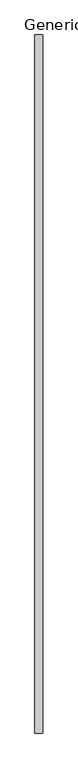
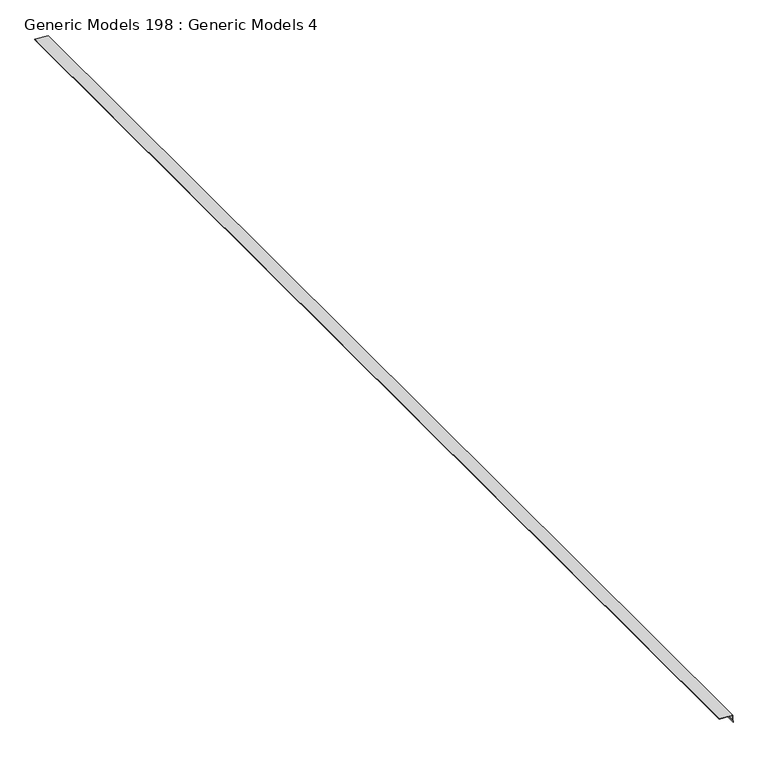
"""IFC4 building model written with IfcOpenShell, lengths in millimetres: proxy geometry, Generic Models 198 : Generic Models 4."""

from ifc_helpers import new_model, si_unit, frame, origin, place, context, project, spatial, polyline, outline, extrude, source, transform, mapped, element, save


def generic_models_198_generic_models_4_338ca49c(model_context):
    return source(origin(), model_context, "Body", "SweptSolid", [
        extrude(outline(polyline([(126852.2693751, -8160.3860198), (126833.2354151, -8160.3860198), (126833.2354151, -8159.5922698), (126852.4093346, -8159.5922698), (126859.5412752, -8162.1880839), (126925.6844476, -8162.1880839), (126932.2834421, -8320.5639511), (126931.4903802, -8320.5969953), (126924.9230818, -8162.9818339), (126859.4013156, -8162.9818339), (126852.2693751, -8160.3860198)])), frame((0.0, -6864.9230338, 0.0), z_axis=(0.0, 1.0, 0.0), x_axis=(0.0, 0.0, 1.0)), (0.0, 0.0, 1.0), 13919.2),
    ])


if __name__ == "__main__":
    model = new_model("IFC4")
    model_context = context("Model", 3, world=origin())
    ifc_project = project(units=[si_unit("LENGTHUNIT", "METRE", prefix="MILLI")], contexts=[model_context])
    site = spatial("IfcSite", under=ifc_project)
    building = spatial("IfcBuilding", under=site)
    placement = place(None, origin())
    generic_models_198_generic_models_4_shape = generic_models_198_generic_models_4_338ca49c(model_context)
    element("IfcBuildingElementProxy", 1, Name="Generic Models 198 : Generic Models 4", ObjectType="Generic Models 198 : Generic Models 4", at=placement, inside=building, context=model_context, shape_type="MappedRepresentation", body=[
        mapped(generic_models_198_generic_models_4_shape, transform((0.0, 0.0, 0.0), x_axis=(1.0, 0.0, 0.0), y_axis=(0.0, 1.0, 0.0), z_axis=(0.0, 0.0, 1.0))),
    ])
    save(model, "model.ifc")

# Revit data of these elements
# Element 1 (IfcBuildingElementProxy, "Generic Models 198 : Generic Models 4")
#   Materials on its faces: "_(2) LAYERS NO. 30 ASTM D226 ASPHALT SATURATED ORGANIC FELT"
# Materials
#   "_(2) LAYERS NO. 30 ASTM D226 ASPHALT SATURATED ORGANIC FELT": class "Generic", colour RGB 67 154 161, transparency 0, Cost = 0
